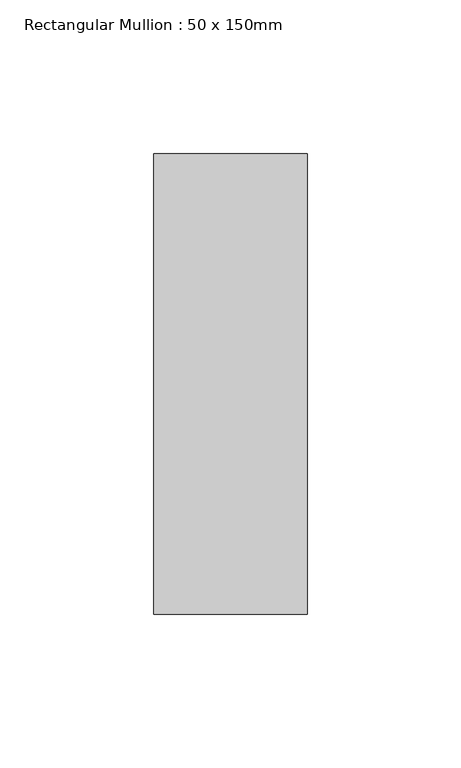
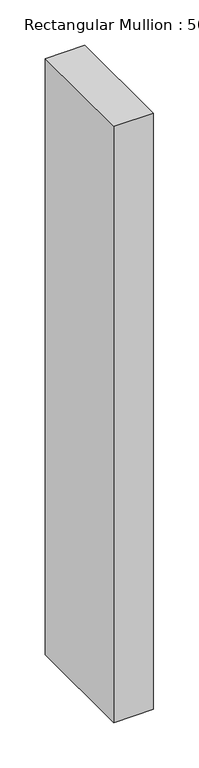
"""IFC4 building model written with IfcOpenShell, lengths in millimetres: member geometry, Rectangular Mullion : 50 x 150mm."""

from ifc_helpers import new_model, si_unit, frame, origin, place, context, project, spatial, polyline, outline, extrude, source, transform, mapped, element, save


def rectangular_mullion_50_x_150mm_6ffebc0f(model_context):
    return source(origin(), model_context, "Body", "SweptSolid", [
        extrude(outline(polyline([(0.0, 75.0), (0.0, -75.0), (-50.0, -75.0), (-50.0, 75.0), (0.0, 75.0)])), frame((0.0, 0.0, -800.0), z_axis=(0.0, 0.0, 1.0), x_axis=(1.0, 0.0, 0.0)), (0.0, 0.0, 1.0), 800.0),
    ])


if __name__ == "__main__":
    model = new_model("IFC4")
    model_context = context("Model", 3, world=origin())
    ifc_project = project(units=[si_unit("LENGTHUNIT", "METRE", prefix="MILLI")], contexts=[model_context])
    site = spatial("IfcSite", under=ifc_project)
    building = spatial("IfcBuilding", under=site)
    placement = place(None, origin())
    rectangular_mullion_50_x_150mm_shape = rectangular_mullion_50_x_150mm_6ffebc0f(model_context)
    element("IfcMember", 1, ObjectType="Rectangular Mullion : 50 x 150mm", at=placement, inside=building, context=model_context, shape_type="MappedRepresentation", body=[
        mapped(rectangular_mullion_50_x_150mm_shape, transform((0.0, 0.0, 0.0), x_axis=(1.0, 0.0, 0.0), y_axis=(0.0, 1.0, 0.0), z_axis=(0.0, 0.0, 1.0))),
    ])
    save(model, "model.ifc")

# Revit data of these elements
# Type "Rectangular Mullion : 50 x 150mm"
#   built-in parameter 1007304 = 0.492126 (stored number, unit not read)
#   built-in parameter 1007301 = 0.082021 (stored number, unit not read)
#   built-in parameter 1007300 = 0.082021 (stored number, unit not read)
# Element 1 (IfcMember, "Rectangular Mullion : 50 x 150mm")
#   Materials on its faces: "Metal - Aluminium"
# Materials
#   "Metal - Aluminium": class "Metal", colour RGB 247 247 247, transparency 0
